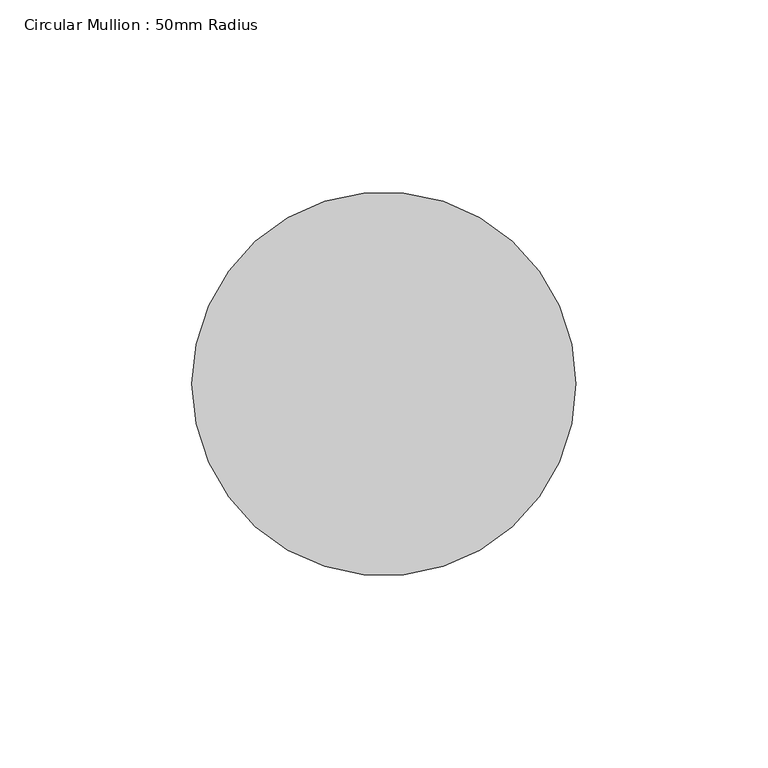
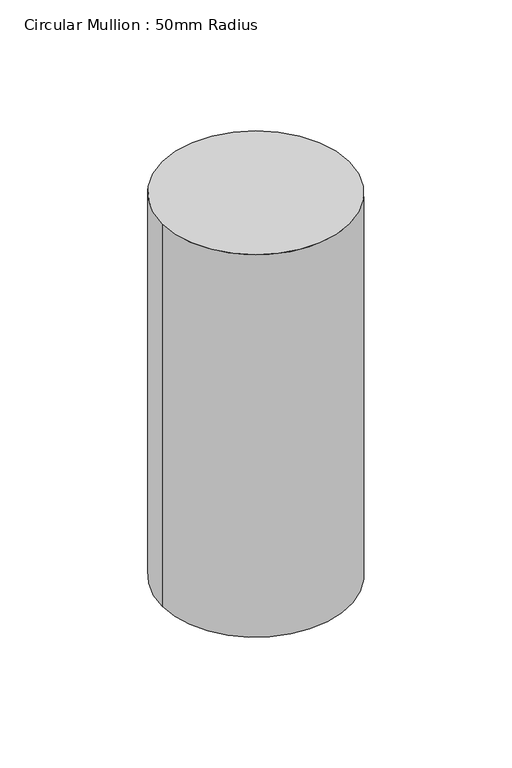
"""IFC4 building model written with IfcOpenShell, lengths in millimetres: member geometry, Circular Mullion : 50mm Radius."""

from ifc_helpers import new_model, si_unit, point, frame, origin, origin_2d, place, context, project, spatial, circle_curve, trimmed, segment, composite_curve, outline, extrude, source, transform, mapped, element, save


def circular_mullion_50mm_radius_230b1f03(model_context):
    return source(origin(), model_context, "Body", "SweptSolid", [
        extrude(outline(composite_curve([segment(trimmed(circle_curve(origin_2d(), 50.0), [point((50.0, 0.0))], [point((-50.0, 0.0))], False, "CARTESIAN"), True, "CONTINUOUS"), segment(trimmed(circle_curve(origin_2d(), 50.0), [point((-50.0, 0.0))], [point((50.0, 0.0))], False, "CARTESIAN"), True, "CONTINUOUS")], self_intersect=False)), frame((0.0, 0.0, -215.9011631), z_axis=(0.0, 0.0, 1.0), x_axis=(1.0, 0.0, 0.0)), (0.0, 0.0, 1.0), 215.9011631),
    ])


if __name__ == "__main__":
    model = new_model("IFC4")
    model_context = context("Model", 3, world=origin())
    ifc_project = project(units=[si_unit("LENGTHUNIT", "METRE", prefix="MILLI")], contexts=[model_context])
    site = spatial("IfcSite", under=ifc_project)
    building = spatial("IfcBuilding", under=site)
    placement = place(None, origin())
    circular_mullion_50mm_radius_shape = circular_mullion_50mm_radius_230b1f03(model_context)
    element("IfcMember", 1, ObjectType="Circular Mullion : 50mm Radius", at=placement, inside=building, context=model_context, shape_type="MappedRepresentation", body=[
        mapped(circular_mullion_50mm_radius_shape, transform((0.0, 0.0, 0.0), x_axis=(1.0, 0.0, 0.0), y_axis=(0.0, 1.0, 0.0), z_axis=(0.0, 0.0, 1.0))),
    ])
    save(model, "model.ifc")

# Revit data of these elements
# Type "Circular Mullion : 50mm Radius"
#   built-in parameter 1007350 = 0.164042 (stored number, unit not read)
# Element 1 (IfcMember, "Circular Mullion : 50mm Radius")
#   Materials on its faces: "Aluminium"
# Materials
#   "Aluminium": class "Metal", colour RGB 247 247 247, transparency 0, Description = "Aluminium 6061", Cost = 0
